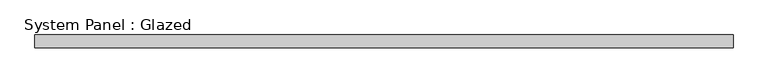
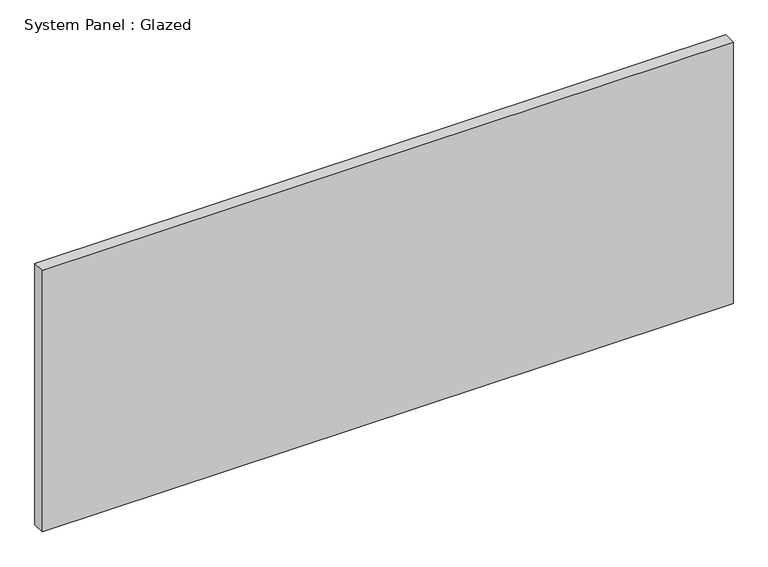
"""IFC4 building model written with IfcOpenShell, lengths in millimetres: plate geometry, System Panel : Glazed."""

from ifc_helpers import new_model, si_unit, origin, origin_with_axes, place, context, project, spatial, polyline, outline, extrude, source, transform, mapped, element, save


def system_panel_glazed_b3b98be9(model_context):
    return source(origin(), model_context, "Body", "SweptSolid", [
        extrude(outline(polyline([(687.25, 24.5), (-687.25, 24.5), (-687.25, 49.5), (687.25, 49.5), (687.25, 24.5)])), origin_with_axes(), (0.0, 0.0, 1.0), 550.0),
    ])


if __name__ == "__main__":
    model = new_model("IFC4")
    model_context = context("Model", 3, world=origin())
    ifc_project = project(units=[si_unit("LENGTHUNIT", "METRE", prefix="MILLI")], contexts=[model_context])
    site = spatial("IfcSite", under=ifc_project)
    building = spatial("IfcBuilding", under=site)
    placement = place(None, origin())
    system_panel_glazed_shape = system_panel_glazed_b3b98be9(model_context)
    element("IfcPlate", 1, ObjectType="System Panel : Glazed", at=placement, inside=building, context=model_context, shape_type="MappedRepresentation", body=[
        mapped(system_panel_glazed_shape, transform((0.0, 0.0, 0.0), x_axis=(1.0, 0.0, 0.0), y_axis=(0.0, 1.0, 0.0), z_axis=(0.0, 0.0, 1.0))),
    ])
    save(model, "model.ifc")

# Revit data of these elements
# Element 1 (IfcPlate, "System Panel : Glazed")
#   Materials on its faces: "Glass"
# Materials
#   "Glass": class "Glass", colour RGB 218 227 224, transparency 0.85, Description = "Soda Lime Glass", Cost = 0
